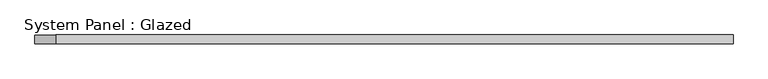
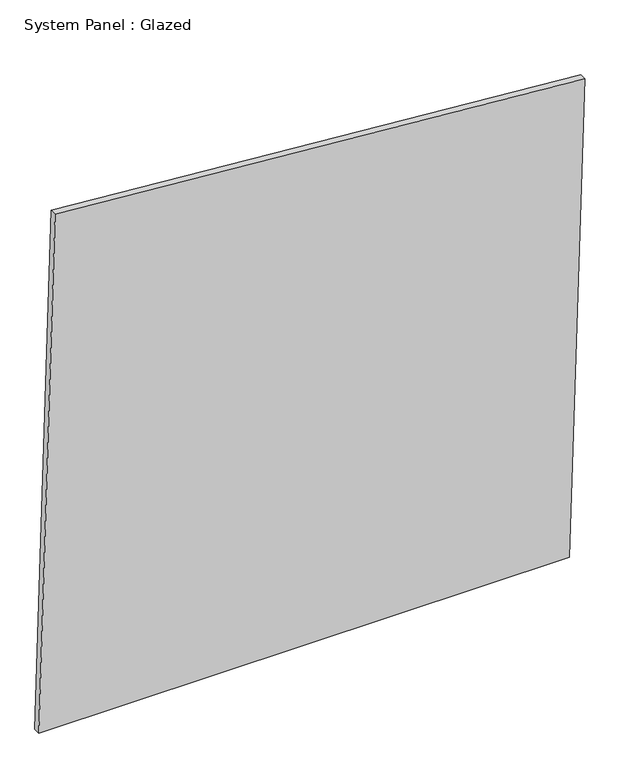
"""IFC4 building model written with IfcOpenShell, lengths in millimetres: plate geometry, System Panel : Glazed."""

from ifc_helpers import new_model, si_unit, frame, origin, place, context, project, spatial, polyline, outline, extrude, source, transform, mapped, element, save


def system_panel_glazed_fa6ac5bb(model_context):
    return source(origin(), model_context, "Body", "SweptSolid", [
        extrude(outline(polyline([(0.0, -1003.6052901), (0.0, 946.2862543), (1838.9863035, 1003.6052901), (1993.8564357, -944.1571371), (0.0, -1003.6052901)])), frame((0.0, -49.5, 0.0), z_axis=(0.0, 1.0, 0.0), x_axis=(0.0, 0.0, 1.0)), (0.0, 0.0, 1.0), 25.0),
    ])


if __name__ == "__main__":
    model = new_model("IFC4")
    model_context = context("Model", 3, world=origin())
    ifc_project = project(units=[si_unit("LENGTHUNIT", "METRE", prefix="MILLI")], contexts=[model_context])
    site = spatial("IfcSite", under=ifc_project)
    building = spatial("IfcBuilding", under=site)
    placement = place(None, origin())
    system_panel_glazed_shape = system_panel_glazed_fa6ac5bb(model_context)
    element("IfcPlate", 1, ObjectType="System Panel : Glazed", at=placement, inside=building, context=model_context, shape_type="MappedRepresentation", body=[
        mapped(system_panel_glazed_shape, transform((0.0, 0.0, 0.0), x_axis=(1.0, 0.0, 0.0), y_axis=(0.0, 1.0, 0.0), z_axis=(0.0, 0.0, 1.0))),
    ])
    save(model, "model.ifc")

# Revit data of these elements
# Element 1 (IfcPlate, "System Panel : Glazed")
#   Materials on its faces: "Glass, Clear Glazing"
# Materials
#   "Glass, Clear Glazing": class "Glass", colour RGB 247 249 248, transparency 0.85, Description = "Clear glazing", Cost = 0
